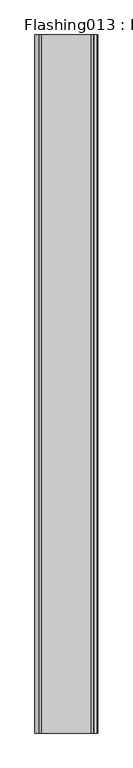
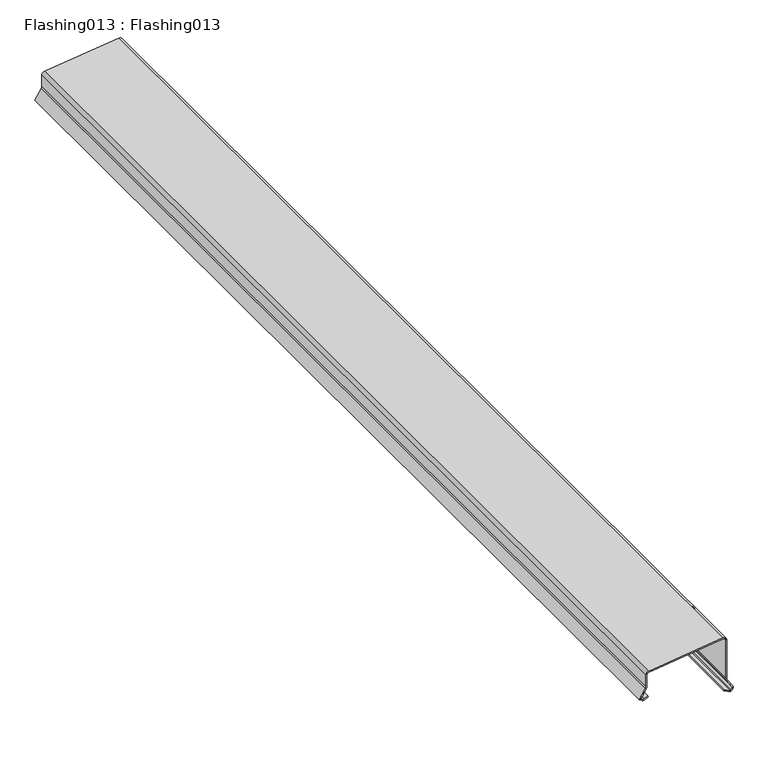
"""IFC4 building model written with IfcOpenShell, lengths in millimetres: proxy geometry, Flashing013 : Flashing013."""

from ifc_helpers import new_model, si_unit, point, frame, frame_2d, origin, place, context, project, spatial, polyline, circle_curve, trimmed, segment, composite_curve, outline, extrude, source, transform, mapped, element, save


def flashing013_flashing013_fca4859d(model_context):
    return source(origin(), model_context, "Body", "SweptSolid", [
        extrude(outline(composite_curve([segment(polyline([(40127.5360053, -9416.8782953), (40130.8867187, -9409.9548736), (40132.6869689, -9410.8261368), (40129.3362554, -9417.7495585)]), True, "CONTINUOUS"), segment(trimmed(circle_curve(frame_2d((40133.2517994, -9419.6445559)), 4.35), [point((40129.3362554, -9417.7495585))], [point((40129.5632143, -9421.9503831))], True, "CARTESIAN"), True, "CONTINUOUS"), segment(polyline([(40129.5632143, -9421.9503831), (40131.5072723, -9425.0602534), (40148.3948046, -9414.1661265)]), True, "CONTINUOUS"), segment(trimmed(circle_curve(frame_2d((40152.9212544, -9421.1828033)), 8.35), [point((40148.3948046, -9414.1661265))], [point((40152.9212544, -9412.8328033))], False, "CARTESIAN"), True, "CONTINUOUS"), segment(polyline([(40152.9212544, -9412.8328033), (40176.1640916, -9412.8328033)]), True, "CONTINUOUS"), segment(trimmed(circle_curve(frame_2d((40176.1640916, -9408.4828033)), 4.35), [point((40176.1640916, -9412.8328033))], [point((40180.4823161, -9409.0076242))], True, "CARTESIAN"), True, "CONTINUOUS"), segment(polyline([(40180.4823161, -9409.0076242), (40197.712243, -9267.2398508)]), True, "CONTINUOUS"), segment(trimmed(circle_curve(frame_2d((40193.3940184, -9266.7150298)), 4.35), [point((40197.712243, -9267.2398508))], [point((40193.3940184, -9262.3650298))], True, "CARTESIAN"), True, "CONTINUOUS"), segment(polyline([(40193.3940184, -9262.3650298), (40116.1659228, -9262.3650299)]), True, "CONTINUOUS"), segment(trimmed(circle_curve(frame_2d((40116.1659228, -9254.0150299)), 8.35), [point((40116.1659228, -9262.3650299))], [point((40111.6503228, -9261.0386939))], False, "CARTESIAN"), True, "CONTINUOUS"), segment(polyline([(40111.6503228, -9261.0386939), (40095.8098632, -9250.8546675)]), True, "CONTINUOUS"), segment(trimmed(circle_curve(frame_2d((40093.4574249, -9254.5137021)), 4.35), [point((40095.8098632, -9250.8546675))], [point((40089.7935443, -9252.1688185))], True, "CARTESIAN"), True, "CONTINUOUS"), segment(polyline([(40089.7935443, -9252.1688185), (40088.63264, -9253.9827315), (40093.9764738, -9264.6739664), (40092.1875, -9265.5681549), (40086.3359375, -9253.8611236), (40088.1090015, -9251.0907111)]), True, "CONTINUOUS"), segment(trimmed(circle_curve(frame_2d((40093.4574249, -9254.5137021)), 6.35), [point((40088.1090015, -9251.0907111))], [point((40096.8914441, -9249.1723528))], False, "CARTESIAN"), True, "CONTINUOUS"), segment(polyline([(40096.8914441, -9249.1723528), (40112.7319037, -9259.3563791)]), True, "CONTINUOUS"), segment(trimmed(circle_curve(frame_2d((40116.1659228, -9254.0150299)), 6.35), [point((40112.7319037, -9259.3563791))], [point((40116.1659228, -9260.3650299))], True, "CARTESIAN"), True, "CONTINUOUS"), segment(polyline([(40116.1659228, -9260.3650299), (40193.3940184, -9260.3650299)]), True, "CONTINUOUS"), segment(trimmed(circle_curve(frame_2d((40193.3940184, -9266.7150299)), 6.35), [point((40193.3940184, -9260.3650299))], [point((40199.6976336, -9267.4811477))], False, "CARTESIAN"), True, "CONTINUOUS"), segment(polyline([(40199.6976336, -9267.4811477), (40182.4677067, -9409.2489212)]), True, "CONTINUOUS"), segment(trimmed(circle_curve(frame_2d((40176.1640916, -9408.4828033)), 6.35), [point((40182.4677067, -9409.2489212))], [point((40176.1640916, -9414.8328033))], False, "CARTESIAN"), True, "CONTINUOUS"), segment(polyline([(40176.1640916, -9414.8328033), (40152.9212544, -9414.8328033)]), True, "CONTINUOUS"), segment(trimmed(circle_curve(frame_2d((40152.9212544, -9421.1828033)), 6.35), [point((40152.9212544, -9414.8328033))], [point((40149.4789842, -9415.8467677))], True, "CARTESIAN"), True, "CONTINUOUS"), segment(polyline([(40149.4789842, -9415.8467677), (40130.8867187, -9427.8406158), (40127.867313, -9423.0105336)]), True, "CONTINUOUS"), segment(trimmed(circle_curve(frame_2d((40133.2517994, -9419.6445559)), 6.35), [point((40127.867313, -9423.0105336))], [point((40127.5360053, -9416.8782953))], False, "CARTESIAN"), True, "CONTINUOUS")], self_intersect=False)), frame((0.0, 7982.1531721, 0.0), z_axis=(0.0, 1.0, 0.0), x_axis=(0.0, 0.0, 1.0)), (0.0, 0.0, 1.0), 2000.0),
    ])


if __name__ == "__main__":
    model = new_model("IFC4")
    model_context = context("Model", 3, world=origin())
    ifc_project = project(units=[si_unit("LENGTHUNIT", "METRE", prefix="MILLI")], contexts=[model_context])
    site = spatial("IfcSite", under=ifc_project)
    building = spatial("IfcBuilding", under=site)
    placement = place(None, origin())
    flashing013_flashing013_shape = flashing013_flashing013_fca4859d(model_context)
    element("IfcBuildingElementProxy", 1, Name="Flashing013 : Flashing013", ObjectType="Flashing013 : Flashing013", at=placement, inside=building, context=model_context, shape_type="MappedRepresentation", body=[
        mapped(flashing013_flashing013_shape, transform((0.0, 0.0, 0.0), x_axis=(1.0, 0.0, 0.0), y_axis=(0.0, 1.0, 0.0), z_axis=(0.0, 0.0, 1.0))),
    ])
    save(model, "model.ifc")

# Revit data of these elements
# Type "Flashing013 : Flashing013"
#   NameOverride = "Flashing013"
# Element 1 (IfcBuildingElementProxy, "Flashing013 : Flashing013")
#   Materials on its faces: "METAL COPING"
# Materials
#   "METAL COPING": class "Unassigned", colour RGB 128 128 128, transparency 0
